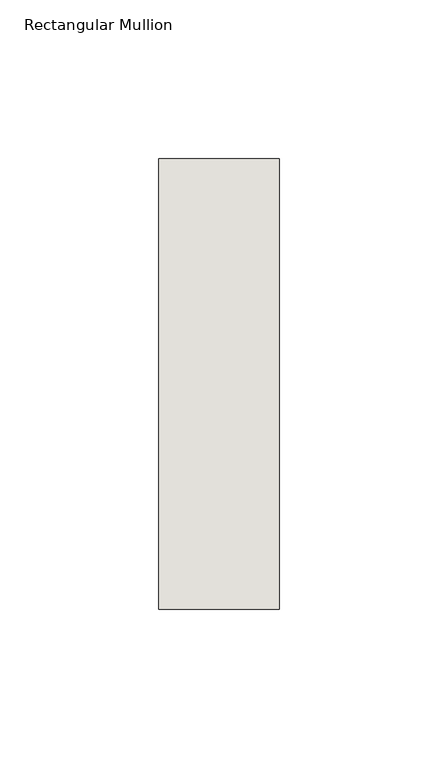
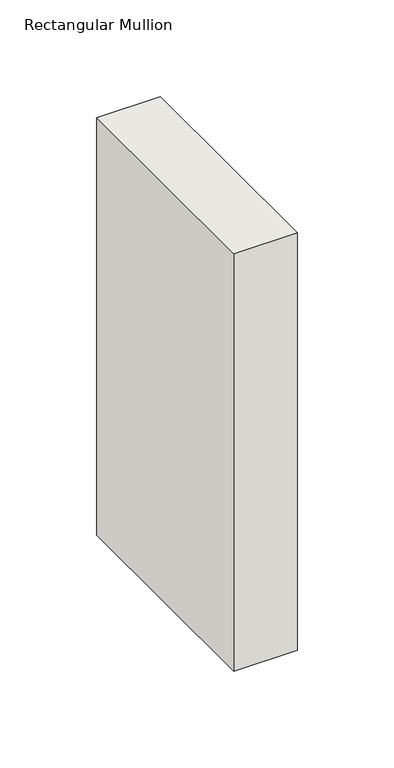
"""IFC4 building model written with IfcOpenShell, lengths in millimetres: wall geometry, Rectangular Mullion : NLRS_21_CWM_hsb-regel 38x142_gen_rsf."""

from ifc_helpers import new_model, si_unit, frame, origin, place, context, project, spatial, polyline, outline, extrude, source, transform, mapped, element, save


def rectangular_mullion_45174ede(model_context):
    return source(origin(), model_context, "Body", "SweptSolid", [
        extrude(outline(polyline([(0.0, -71.0), (-38.0, -71.0), (-38.0, 71.0), (0.0, 71.0), (0.0, -71.0)])), frame((0.0, 0.0, -264.0000003), z_axis=(0.0, 0.0, 1.0), x_axis=(1.0, 0.0, 0.0)), (0.0, 0.0, 1.0), 264.0000003),
    ])


if __name__ == "__main__":
    model = new_model("IFC4")
    model_context = context("Model", 3, world=origin())
    ifc_project = project(units=[si_unit("LENGTHUNIT", "METRE", prefix="MILLI")], contexts=[model_context])
    site = spatial("IfcSite", under=ifc_project)
    building = spatial("IfcBuilding", under=site)
    placement = place(None, origin())
    rectangular_mullion_shape = rectangular_mullion_45174ede(model_context)
    element("IfcWall", 1, ObjectType="Rectangular Mullion : NLRS_21_CWM_hsb-regel 38x142_gen_rsf", at=placement, inside=building, context=model_context, shape_type="MappedRepresentation", body=[
        mapped(rectangular_mullion_shape, transform((0.0, 0.0, 0.0), x_axis=(1.0, 0.0, 0.0), y_axis=(0.0, 1.0, 0.0), z_axis=(0.0, 0.0, 1.0))),
    ])
    save(model, "model.ifc")

# Revit data of these elements
# Type "Rectangular Mullion : NLRS_21_CWM_hsb-regel 38x142_gen_rsf"
#   Type IfcGUID = "07M7mRoiH1CR8m_RSKIwpF"
#   Assembly Code = "21.10"
#   IfcExportAs = "IfcWall"
#   built-in parameter 1007322 = 0.465879 (stored number, unit not read)
#   built-in parameter 1007321 = 0.062336 (stored number, unit not read)
#   built-in parameter 1007320 = 0.062336 (stored number, unit not read)
# Element 1 (IfcWall, "Rectangular Mullion : NLRS_21_CWM_hsb-regel 38x142_gen_rsf")
#   Materials on its faces: "NLRS_i2_hout naaldhout vuren_gen_rsf"
# Materials
#   "NLRS_i2_hout naaldhout vuren_gen_rsf": class "I - Hout", colour RGB 234 199 147, transparency 0, Keynote = "i2", Manufacturer = "Revit Standards Foundation", URL = "www.revitstandards.org", Description = "hout vuren", Cost = 0
